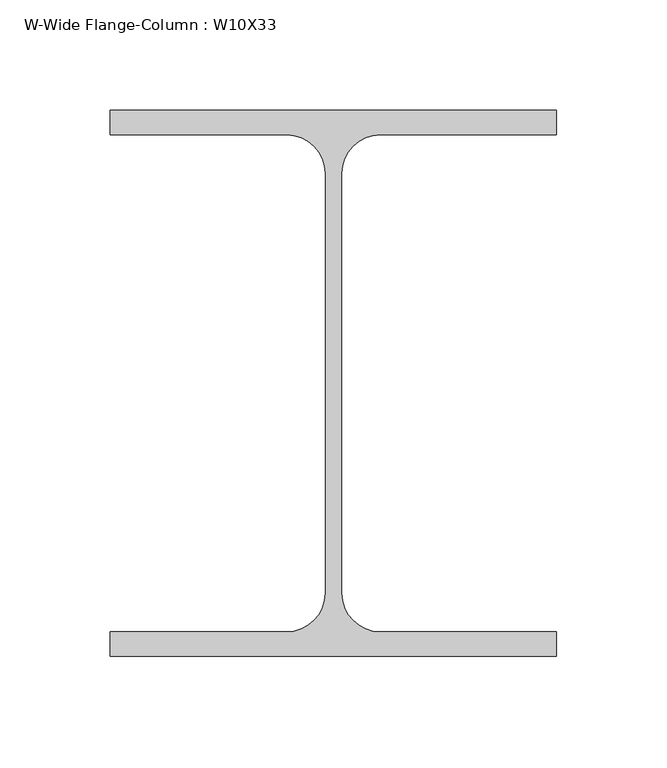
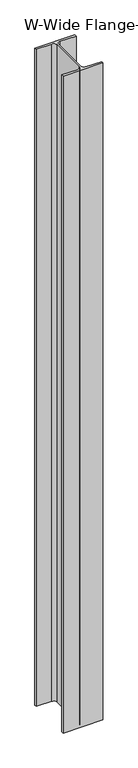
"""IFC4 building model written with IfcOpenShell, lengths in millimetres: column geometry, W-Wide Flange-Column : W10X33."""

import ifcopenshell
import ifcopenshell.guid

model = None  # the IFC model being written
_history = None  # IfcOwnerHistory: only IFC2X3 demands one
_inside = {}  # id of a spatial element -> (the spatial element, [elements in it])
_under = {}  # id of a project, library or spatial element -> (it, [spatial elements below it])
_declared = {}  # id of a project -> (the project, [libraries it declares])
_typed = {}  # id of a type object -> (the type object, [elements of that type])
_made_of = {}  # id of a material, layer set ... -> (it, [elements and type objects made of it])


def new_model(schema):
    """Start an empty IFC model of exactly this schema.

    Asked for "IFC4X3", IfcOpenShell would pick the latest addendum, in which some entities
    have other attributes; the version numbers below select the first issue.
    IFC2X3 requires an IfcOwnerHistory on every rooted entity: one is made here for all.
    """
    global model, _history
    if schema == "IFC4X3":
        model = ifcopenshell.file(schema_version=(4, 3, 0, 0))
    else:
        model = ifcopenshell.file(schema=schema)
    _inside.clear()
    _under.clear()
    _declared.clear()
    _typed.clear()
    _made_of.clear()
    _history = None
    if model.schema == "IFC2X3":
        org = make("IfcOrganization", Name="unknown")
        user = make(
            "IfcPersonAndOrganization",
            ThePerson=make("IfcPerson", FamilyName="unknown"),
            TheOrganization=org,
        )
        app = make(
            "IfcApplication",
            ApplicationDeveloper=org,
            Version="unknown",
            ApplicationFullName="unknown",
            ApplicationIdentifier="unknown",
        )
        _history = make(
            "IfcOwnerHistory",
            OwningUser=user,
            OwningApplication=app,
            ChangeAction="ADDED",
            CreationDate=0,
        )
    return model


def make(cls, **values):
    """One entity of the class cls with the attributes given. An attribute that is None is left unset."""
    return model.create_entity(
        cls, **{name: value for name, value in values.items() if value is not None}
    )


def rooted(cls, **values):
    """An entity with a GlobalId (a new one), such as an element, a storey or a relation."""
    return make(cls, GlobalId=ifcopenshell.guid.new(), OwnerHistory=_history, **values)


def si_unit(unit_type, name, prefix=None):
    """IfcSIUnit, for example si_unit("LENGTHUNIT", "METRE", prefix="MILLI")."""
    return make("IfcSIUnit", UnitType=unit_type, Prefix=prefix, Name=name)


def assignment(units):
    """IfcUnitAssignment: the units of a project."""
    return None if units is None else make("IfcUnitAssignment", Units=units)


def point(xyz):
    """IfcCartesianPoint."""
    return None if xyz is None else make("IfcCartesianPoint", Coordinates=xyz)


def direction(xyz):
    """IfcDirection."""
    return None if xyz is None else make("IfcDirection", DirectionRatios=xyz)


def frame(location, z_axis=None, x_axis=None):
    """IfcAxis2Placement3D, a coordinate frame: its origin and axes. An axis left out is left unset."""
    return make(
        "IfcAxis2Placement3D",
        Location=point(location),
        Axis=direction(z_axis),
        RefDirection=direction(x_axis),
    )


def frame_2d(location, x_axis=None):
    """IfcAxis2Placement2D, a coordinate frame in the plane: its origin and x axis."""
    return make(
        "IfcAxis2Placement2D", Location=point(location), RefDirection=direction(x_axis)
    )


def origin():
    """The frame at (0, 0, 0) with its axes left unset."""
    return frame((0.0, 0.0, 0.0))


def place(relative_to, where):
    """IfcLocalPlacement: puts the frame where relative to a parent placement (None: the world)."""
    return make(
        "IfcLocalPlacement", PlacementRelTo=relative_to, RelativePlacement=where
    )


def context(
    kind, dimensions, precision=None, world=None, true_north=None, identifier=None
):
    """IfcGeometricRepresentationContext, for example the 3D "Model" context."""
    return make(
        "IfcGeometricRepresentationContext",
        ContextIdentifier=identifier,
        ContextType=kind,
        CoordinateSpaceDimension=dimensions,
        Precision=precision,
        WorldCoordinateSystem=world,
        TrueNorth=true_north,
    )


def project(units=None, contexts=None):
    """IfcProject with its units and contexts."""
    return rooted(
        "IfcProject",
        Name="project",
        RepresentationContexts=contexts,
        UnitsInContext=assignment(units),
    )


def spatial(cls, under=None, at=None, **own):
    """A site, building, storey or space (cls), placed at a placement, below another one or the project."""
    s = rooted(cls, ObjectPlacement=at, **own)
    if under is not None:
        _under.setdefault(under.id(), (under, []))[1].append(s)
    return s


def polyline(points):
    """IfcPolyline through the points."""
    return make("IfcPolyline", Points=[point(p) for p in points])


def circle_curve(where, radius):
    """IfcCircle in the frame where."""
    return make("IfcCircle", Position=where, Radius=radius)


def trimmed(basis, trim1, trim2, sense, master):
    """IfcTrimmedCurve: the piece of a basis curve between two trims."""
    return make(
        "IfcTrimmedCurve",
        BasisCurve=basis,
        Trim1=trim1,
        Trim2=trim2,
        SenseAgreement=sense,
        MasterRepresentation=master,
    )


def segment(curve, same_sense, transition):
    """IfcCompositeCurveSegment."""
    return make(
        "IfcCompositeCurveSegment",
        Transition=transition,
        SameSense=same_sense,
        ParentCurve=curve,
    )


def composite_curve(segments, self_intersect=None):
    """IfcCompositeCurve: segments joined end to end."""
    return make("IfcCompositeCurve", Segments=segments, SelfIntersect=self_intersect)


def outline(outer, holes=None, kind="AREA"):
    """IfcArbitraryClosedProfileDef: a profile drawn as a closed curve; with holes, ...WithVoids."""
    if holes is None:
        return make("IfcArbitraryClosedProfileDef", ProfileType=kind, OuterCurve=outer)
    return make(
        "IfcArbitraryProfileDefWithVoids",
        ProfileType=kind,
        OuterCurve=outer,
        InnerCurves=holes,
    )


def extrude(swept, where, along, depth):
    """IfcExtrudedAreaSolid: the profile swept, set in the frame where, extruded along a direction by depth."""
    return make(
        "IfcExtrudedAreaSolid",
        SweptArea=swept,
        Position=where,
        ExtrudedDirection=direction(along),
        Depth=depth,
    )


def shape(context_of_items, identifier, shape_type, items):
    """IfcShapeRepresentation: the items that make up one representation, for example the "Body"."""
    return make(
        "IfcShapeRepresentation",
        ContextOfItems=context_of_items,
        RepresentationIdentifier=identifier,
        RepresentationType=shape_type,
        Items=items,
    )


def source(mapping_origin, context_of_items, identifier, shape_type, items):
    """IfcRepresentationMap: a shape defined once, which mapped items show again and again."""
    return make(
        "IfcRepresentationMap",
        MappingOrigin=mapping_origin,
        MappedRepresentation=shape(context_of_items, identifier, shape_type, items),
    )


def transform(
    local_origin,
    x_axis=None,
    y_axis=None,
    z_axis=None,
    scale=None,
    scale2=None,
    scale3=None,
    uniform=True,
):
    """IfcCartesianTransformationOperator3D, or its non-uniform kind. x_axis, y_axis, z_axis: its Axis1, 2, 3."""
    if uniform:
        return make(
            "IfcCartesianTransformationOperator3D",
            Axis1=direction(x_axis),
            Axis2=direction(y_axis),
            LocalOrigin=point(local_origin),
            Scale=scale,
            Axis3=direction(z_axis),
        )
    return make(
        "IfcCartesianTransformationOperator3DnonUniform",
        Axis1=direction(x_axis),
        Axis2=direction(y_axis),
        LocalOrigin=point(local_origin),
        Scale=scale,
        Axis3=direction(z_axis),
        Scale2=scale2,
        Scale3=scale3,
    )


def mapped(mapping_source, mapping_target):
    """IfcMappedItem: shows the shape of a source again, moved by a transform."""
    return make(
        "IfcMappedItem", MappingSource=mapping_source, MappingTarget=mapping_target
    )


def made_of(thing, what):
    """Note that an element or type object is made of a material, layer set ...; save() writes the relation."""
    if what is not None:
        _made_of.setdefault(what.id(), (what, []))[1].append(thing)
    return thing


def element(
    cls,
    number,
    at=None,
    inside=None,
    cuts=None,
    type_object=None,
    material=None,
    context=None,
    identifier="Body",
    shape_type=None,
    held_by="IfcProductDefinitionShape",
    body=None,
    shapes=None,
    **own,
):
    """One element of the class cls, such as IfcWall. Its Tag is "e" and its number.

    at: its placement. inside: the storey or other place that contains it. cuts: it is an
    opening in that element (IfcRelVoidsElement). A single representation is given by context,
    identifier, shape_type and body (its items); several are given by shapes. held_by: the class
    of the entity that holds the representations. save() writes the other relations.
    """
    e = rooted(cls, Tag="e%d" % number, ObjectPlacement=at, **own)
    if body is not None:
        shapes = [shape(context, identifier, shape_type, body)]
    if shapes is not None:
        e.Representation = make(held_by, Representations=shapes)
    if inside is not None:
        _inside.setdefault(inside.id(), (inside, []))[1].append(e)
    if cuts is not None:
        rooted(
            "IfcRelVoidsElement", RelatingBuildingElement=cuts, RelatedOpeningElement=e
        )
    if type_object is not None:
        _typed.setdefault(type_object.id(), (type_object, []))[1].append(e)
    return made_of(e, material)


def aggregate(whole, parts):
    """IfcRelAggregates: a whole, such as a stair, and the parts it consists of."""
    return rooted("IfcRelAggregates", RelatingObject=whole, RelatedObjects=parts)


def save(model, path):
    """Write the relations noted so far, then the file.

    IfcRelAggregates (storeys below a building ...), IfcRelContainedInSpatialStructure (elements
    in a storey), IfcRelDefinesByType, IfcRelAssociatesMaterial and IfcRelDeclares: one each for
    every whole, place, type object, material and project.
    """
    for whole, parts in _under.values():
        aggregate(whole, parts)
    for where, things in _inside.values():
        rooted(
            "IfcRelContainedInSpatialStructure",
            RelatedElements=things,
            RelatingStructure=where,
        )
    for kind, things in _typed.values():
        rooted("IfcRelDefinesByType", RelatedObjects=things, RelatingType=kind)
    for what, things in _made_of.values():
        rooted("IfcRelAssociatesMaterial", RelatedObjects=things, RelatingMaterial=what)
    for by, libraries in _declared.values():
        rooted("IfcRelDeclares", RelatingContext=by, RelatedDefinitions=libraries)
    model.write(path)


def w_wide_flange_column_w10x33_f4179dd2(model_context):
    return source(origin(), model_context, "Body", "SweptSolid", [
        extrude(outline(composite_curve([segment(polyline([(101.092, 123.571), (101.092, 112.522), (21.209, 112.522)]), True, "CONTINUOUS"), segment(trimmed(circle_curve(frame_2d((21.209, 94.996)), 17.526), [point((21.209, 112.522))], [point((3.683, 94.996))], True, "CARTESIAN"), True, "CONTINUOUS"), segment(polyline([(3.683, 94.996), (3.683, -94.996)]), True, "CONTINUOUS"), segment(trimmed(circle_curve(frame_2d((21.209, -94.996)), 17.526), [point((3.683, -94.996))], [point((21.209, -112.522))], True, "CARTESIAN"), True, "CONTINUOUS"), segment(polyline([(21.209, -112.522), (101.092, -112.522), (101.092, -123.571), (-101.092, -123.571), (-101.092, -112.522), (-21.209, -112.522)]), True, "CONTINUOUS"), segment(trimmed(circle_curve(frame_2d((-21.209, -94.996)), 17.526), [point((-21.209, -112.522))], [point((-3.683, -94.996))], True, "CARTESIAN"), True, "CONTINUOUS"), segment(polyline([(-3.683, -94.996), (-3.683, 94.996)]), True, "CONTINUOUS"), segment(trimmed(circle_curve(frame_2d((-21.209, 94.996)), 17.526), [point((-3.683, 94.996))], [point((-21.209, 112.522))], True, "CARTESIAN"), True, "CONTINUOUS"), segment(polyline([(-21.209, 112.522), (-101.092, 112.522), (-101.092, 123.571), (101.092, 123.571)]), True, "CONTINUOUS")], self_intersect=False)), frame((0.0, 0.0, 8655.05), z_axis=(0.0, 0.0, 1.0), x_axis=(1.0, 0.0, 0.0)), (0.0, 0.0, 1.0), 3524.25),
    ])


if __name__ == "__main__":
    model = new_model("IFC4")
    model_context = context("Model", 3, world=origin())
    ifc_project = project(units=[si_unit("LENGTHUNIT", "METRE", prefix="MILLI")], contexts=[model_context])
    site = spatial("IfcSite", under=ifc_project)
    building = spatial("IfcBuilding", under=site)
    placement = place(None, origin())
    w_wide_flange_column_w10x33_shape = w_wide_flange_column_w10x33_f4179dd2(model_context)
    element("IfcColumn", 1, ObjectType="W-Wide Flange-Column : W10X33", at=placement, inside=building, context=model_context, shape_type="MappedRepresentation", body=[
        mapped(w_wide_flange_column_w10x33_shape, transform((0.0, 0.0, 0.0), x_axis=(1.0, 0.0, 0.0), y_axis=(0.0, 1.0, 0.0), z_axis=(0.0, 0.0, 1.0))),
    ])
    save(model, "model.ifc")

# Revit data of these elements
# Type "W-Wide Flange-Column : W10X33"
#   Assembly Code = "B10"
#   W = 33
#   bf = 0' - 7.96"
#   d = 0' - 9.73"
#   k = 0' - 1 1/8"
#   kr = 0' - 0.69"
#   tf = 0' - 0.435"
#   tw = 0' - 0.29"
#   A = 0.0674306 SF
#   Structural Material [instance default] = Steel ASTM A992
# Element 1 (IfcColumn, "W-Wide Flange-Column : W10X33")
#   Materials on its faces: "Steel ASTM A992"
# Materials
#   "Steel ASTM A992": class "Metal", colour RGB 199 199 199, transparency 0, Description = "Structural steel 50ksi", Cost = 0
